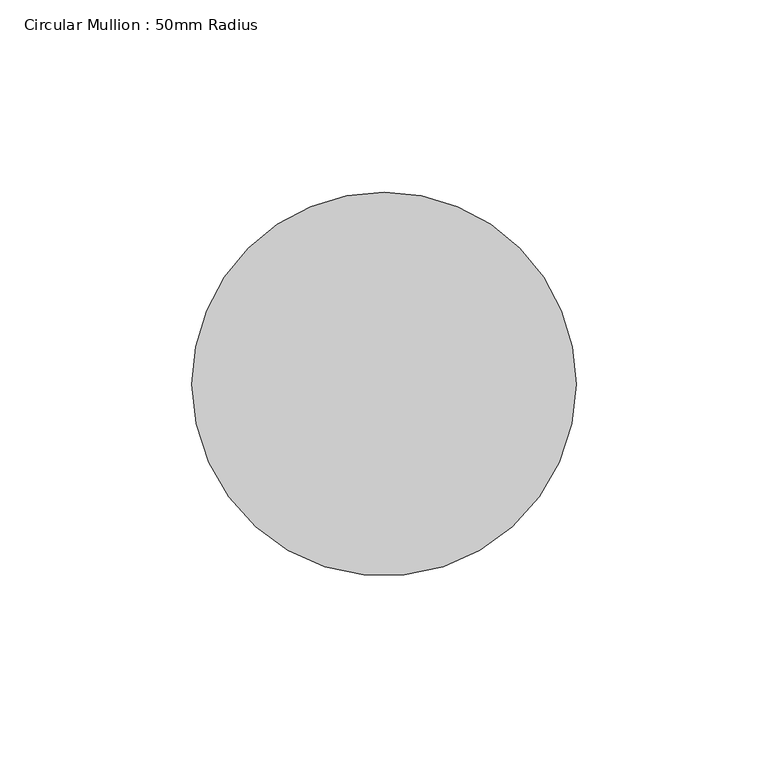
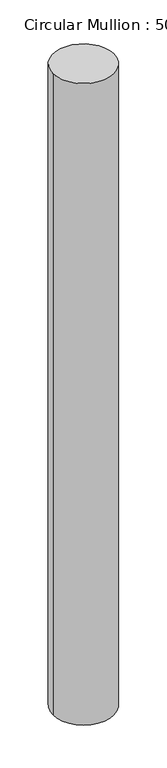
"""IFC4 building model written with IfcOpenShell, lengths in millimetres: member geometry, Circular Mullion : 50mm Radius."""

from ifc_helpers import new_model, si_unit, frame, origin, place, context, project, spatial, ellipse_curve, source, transform, mapped, element, save
from ifc_brep_helpers import plane_surface, cylinder_surface, advanced_brep


def circular_mullion_50mm_radius_11294946(model_context):
    return source(origin(), model_context, "Body", "AdvancedBrep", [
        advanced_brep(
        [(-100.0, 0.0, 1.0969067), (0.0, 0.0, 0.0), (0.0, 0.0, -1103.5496934), (-100.0, 0.0, -1104.68369)],
        [
            (0, 1, ellipse_curve(frame((-50.0, 0.0, 0.5484533), z_axis=(-0.010967187295404825, -0.014910913556380448, -0.9998286780542662), x_axis=(-0.5924039624189791, -0.8054284144292615, 0.01850984981728608)), 50.0085676, 50.0)),
            (1, 2),
            (2, 3, ellipse_curve(frame((-50.0, 0.0, -1104.1166917), z_axis=(-0.011337889515750153, -0.015414917784068005, 0.9998168995226271), x_axis=(0.5923969835745403, 0.805418926039626, 0.019135501795382294)), 50.0091567, 50.0)),
            (3, 0),
            (1, 0, ellipse_curve(frame((-50.0, 0.0, 0.5484533), z_axis=(-0.010967187295404825, -0.014910913556380448, -0.9998286780542662), x_axis=(-0.5924039624189791, -0.8054284144292615, 0.01850984981728608)), 50.0085676, 50.0)),
            (3, 2, ellipse_curve(frame((-50.0, 0.0, -1104.1166917), z_axis=(-0.011337889515750153, -0.015414917784068005, 0.9998168995226271), x_axis=(0.5923969835745403, 0.805418926039626, 0.019135501795382294)), 50.0091567, 50.0)),
        ],
        [
            cylinder_surface(frame((-50.0, 0.0, 0.0), z_axis=(0.0, 0.0, 1.0), x_axis=(1.0, 0.0, 0.0)), 50.0),
            plane_surface(frame((-245.5366465, 180.5956677, 0.0), z_axis=(0.010967187295404827, 0.014910913556380452, 0.9998286780542665), x_axis=(0.5924039624189776, 0.8054284144292628, -0.01850984981728213))),
            plane_surface(frame((-245.5366465, 180.5956677, -1103.5496934), z_axis=(0.011337889515750155, 0.015414917784068009, -0.9998168995226273), x_axis=(0.5923969835745404, 0.8054189260396263, 0.019135501795378488))),
        ],
        [
            (0, [[1, 2, 3, 4]]),
            (0, [[5, -4, 6, -2]]),
            (1, [[-1, -5]]),
            (2, [[-6, -3]]),
        ],
    ),
    ])


if __name__ == "__main__":
    model = new_model("IFC4")
    model_context = context("Model", 3, world=origin())
    ifc_project = project(units=[si_unit("LENGTHUNIT", "METRE", prefix="MILLI")], contexts=[model_context])
    site = spatial("IfcSite", under=ifc_project)
    building = spatial("IfcBuilding", under=site)
    placement = place(None, origin())
    circular_mullion_50mm_radius_shape = circular_mullion_50mm_radius_11294946(model_context)
    element("IfcMember", 1, ObjectType="Circular Mullion : 50mm Radius", at=placement, inside=building, context=model_context, shape_type="MappedRepresentation", body=[
        mapped(circular_mullion_50mm_radius_shape, transform((0.0, 0.0, 0.0), x_axis=(1.0, 0.0, 0.0), y_axis=(0.0, 1.0, 0.0), z_axis=(0.0, 0.0, 1.0))),
    ])
    save(model, "model.ifc")

# Revit data of these elements
# Type "Circular Mullion : 50mm Radius"
#   built-in parameter 1007350 = 0.164042 (stored number, unit not read)
# Element 1 (IfcMember, "Circular Mullion : 50mm Radius")
#   Materials on its faces: "Aluminium"
# Materials
#   "Aluminium": class "Metal", colour RGB 247 247 247, transparency 0, Description = "Aluminium 6061", Cost = 0
